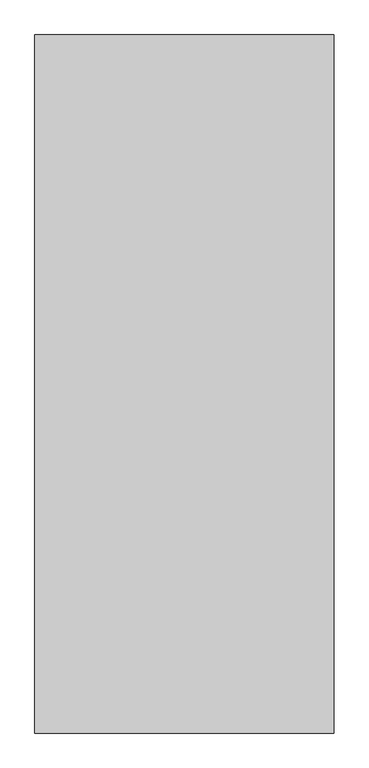
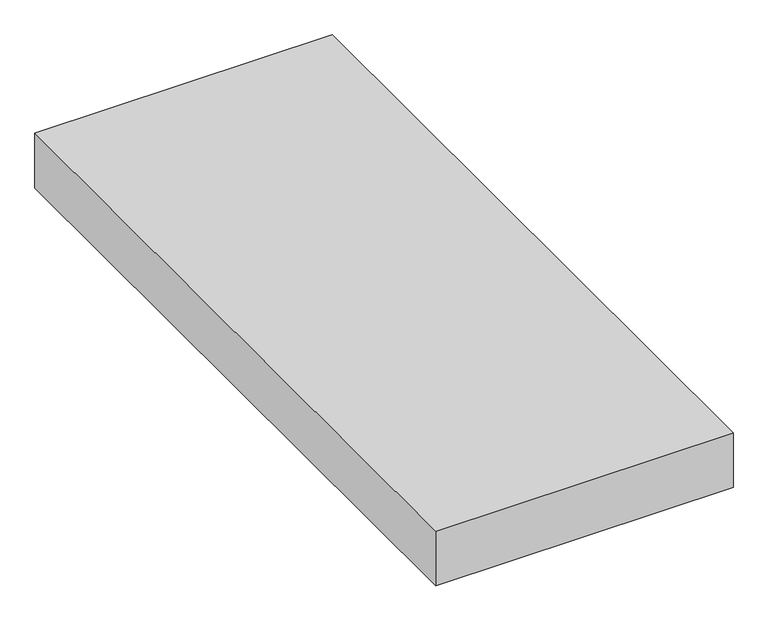
"""IFC4 building model written with IfcOpenShell, lengths in millimetres: proxy geometry, Space Planning Box_hec : Space Planning Box_hec."""

from ifc_helpers import new_model, si_unit, origin, origin_with_axes, place, context, project, spatial, polyline, outline, extrude, source, transform, mapped, element, save


def generic_models_bb515c93(model_context):
    return source(origin(), model_context, "Body", "SweptSolid", [
        extrude(outline(polyline([(9000.0, 21000.0), (9000.0, -21000.0), (-9000.0, -21000.0), (-9000.0, 21000.0), (9000.0, 21000.0)])), origin_with_axes(), (0.0, 0.0, 1.0), 3500.0),
    ])


if __name__ == "__main__":
    model = new_model("IFC4")
    model_context = context("Model", 3, world=origin())
    ifc_project = project(units=[si_unit("LENGTHUNIT", "METRE", prefix="MILLI")], contexts=[model_context])
    site = spatial("IfcSite", under=ifc_project)
    building = spatial("IfcBuilding", under=site)
    placement = place(None, origin())
    generic_models_shape = generic_models_bb515c93(model_context)
    element("IfcBuildingElementProxy", 1, Name="Space Planning Box_hec : Space Planning Box_hec", ObjectType="Space Planning Box_hec : Space Planning Box_hec", at=placement, inside=building, context=model_context, shape_type="MappedRepresentation", body=[
        mapped(generic_models_shape, transform((0.0, 0.0, 0.0), x_axis=(1.0, 0.0, 0.0), y_axis=(0.0, 1.0, 0.0), z_axis=(0.0, 0.0, 1.0))),
    ])
    save(model, "model.ifc")

# Revit data of these elements
# Type "Space Planning Box_hec : Space Planning Box_hec"
#   Type Comments = "..."
#   Room Name [instance default] = "?"
#   Interior Finish [instance default] = ""
#   Exterior Finish [instance default] = ""
#   Department [instance default] = ""
#   Assembly Code = "..."
#   ceiling height [instance default] = 0
#   Width [instance default] = 1524 mm
#   Program Area [instance default] = 0.00 m²
#   Length [instance default] = 1524 mm
#   Height [instance default] = 1524 mm
#   Area [instance default] = 2.32258 m²
#   Fill Color [instance default] = Cyan
#   Default Elevation = 0
# Element 1 (IfcBuildingElementProxy, "Space Planning Box_hec : Space Planning Box_hec")
#   Room Name = "Cable Room"
#   Exterior Finish = "N/A..N/A,,EW1..EW2..N/A"
#   Department = "EL"
#   Width = 18000 mm
#   Program Area = 720.00 m²
#   Length = 42000 mm
#   Height = 3500 mm
#   Area = 756.00 m²
#   Fill Color = Orange
#   Materials on its faces: "Orange"
# Materials
#   "Cyan": class "Generic", colour RGB 0 255 255, transparency 0.2, Cost = 0
#   "Orange": class "Generic", colour RGB 255 165 0, transparency 0.2, Cost = 0
